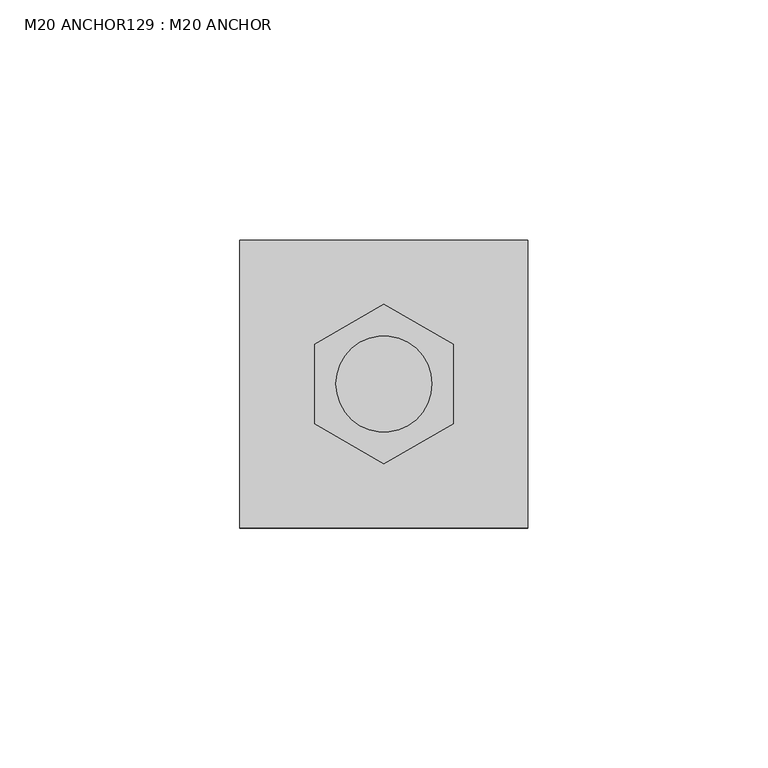
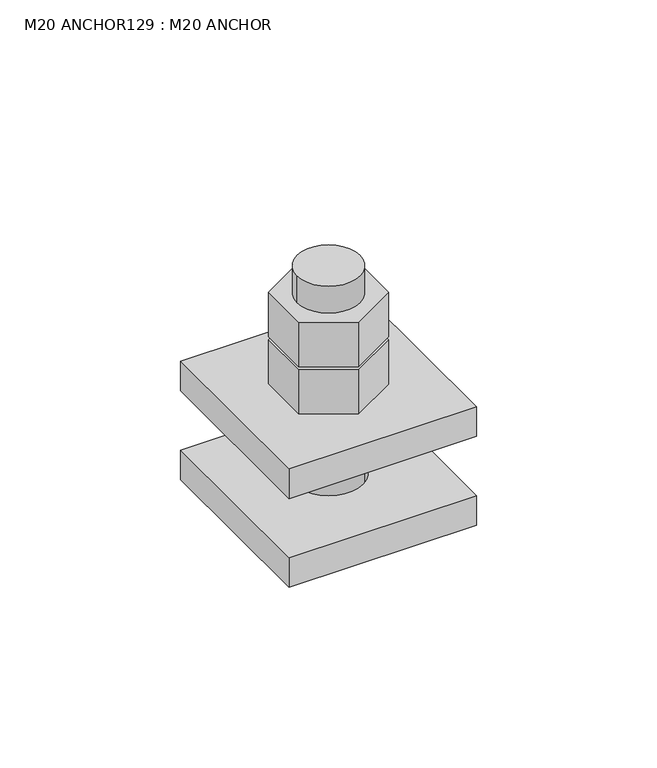
"""IFC4 building model written with IfcOpenShell, lengths in millimetres: fastener geometry, M20 ANCHOR129 : M20 ANCHOR."""

from ifc_helpers import new_model, si_unit, point, frame, frame_2d, origin, place, context, project, spatial, polyline, circle_curve, trimmed, segment, composite_curve, outline, extrude, source, transform, mapped, element, save


def m20_anchor129_m20_anchor_66062f94(model_context):
    return source(origin(), model_context, "Body", "SweptSolid", [
        extrude(outline(polyline([(5991.9144032, 19453.9464399), (5977.5062842, 19445.6279085), (5963.0981652, 19453.9464399), (5963.0981652, 19470.5835027), (5977.5062842, 19478.9020341), (5991.9144032, 19470.5835027), (5991.9144032, 19453.9464399)]), holes=[composite_curve([segment(trimmed(circle_curve(frame_2d((5977.5062842, 19462.2649713)), 10.0), [point((5967.5062842, 19462.2649713))], [point((5987.5062842, 19462.2649713))], True, "CARTESIAN"), True, "CONTINUOUS"), segment(trimmed(circle_curve(frame_2d((5977.5062842, 19462.2649713)), 10.0), [point((5987.5062842, 19462.2649713))], [point((5967.5062842, 19462.2649713))], True, "CARTESIAN"), True, "CONTINUOUS")], self_intersect=False)]), frame((0.0, 0.0, 246.0), z_axis=(0.0, 0.0, 1.0), x_axis=(1.0, 0.0, 0.0)), (0.0, 0.0, 1.0), 15.0),
        extrude(outline(polyline([(5991.9144032, 19453.9464399), (5977.5062842, 19445.6279085), (5963.0981652, 19453.9464399), (5963.0981652, 19470.5835027), (5977.5062842, 19478.9020341), (5991.9144032, 19470.5835027), (5991.9144032, 19453.9464399)]), holes=[composite_curve([segment(trimmed(circle_curve(frame_2d((5977.5062842, 19462.2649713)), 10.0), [point((5967.5062842, 19462.2649713))], [point((5987.5062842, 19462.2649713))], True, "CARTESIAN"), True, "CONTINUOUS"), segment(trimmed(circle_curve(frame_2d((5977.5062842, 19462.2649713)), 10.0), [point((5987.5062842, 19462.2649713))], [point((5967.5062842, 19462.2649713))], True, "CARTESIAN"), True, "CONTINUOUS")], self_intersect=False)]), frame((0.0, 0.0, 230.0), z_axis=(0.0, 0.0, 1.0), x_axis=(1.0, 0.0, 0.0)), (0.0, 0.0, 1.0), 15.0),
        extrude(outline(composite_curve([segment(trimmed(circle_curve(frame_2d((5977.5062842, 19462.2649713)), 10.0), [point((5967.5062842, 19462.2649713))], [point((5987.5062842, 19462.2649713))], False, "CARTESIAN"), True, "CONTINUOUS"), segment(trimmed(circle_curve(frame_2d((5977.5062842, 19462.2649713)), 10.0), [point((5987.5062842, 19462.2649713))], [point((5967.5062842, 19462.2649713))], False, "CARTESIAN"), True, "CONTINUOUS")], self_intersect=False)), frame((0.0, 0.0, 190.0), z_axis=(0.0, 0.0, 1.0), x_axis=(1.0, 0.0, 0.0)), (0.0, 0.0, 1.0), 80.0),
        extrude(outline(polyline([(6007.5062842, 19432.2649713), (5947.5062842, 19432.2649713), (5947.5062842, 19492.2649713), (6007.5062842, 19492.2649713), (6007.5062842, 19432.2649713)]), holes=[composite_curve([segment(trimmed(circle_curve(frame_2d((5977.5062842, 19462.2649713)), 11.0), [point((5966.5062842, 19462.2649713))], [point((5988.5062842, 19462.2649713))], True, "CARTESIAN"), True, "CONTINUOUS"), segment(trimmed(circle_curve(frame_2d((5977.5062842, 19462.2649713)), 11.0), [point((5988.5062842, 19462.2649713))], [point((5966.5062842, 19462.2649713))], True, "CARTESIAN"), True, "CONTINUOUS")], self_intersect=False)]), frame((0.0, 0.0, 190.0), z_axis=(0.0, 0.0, 1.0), x_axis=(1.0, 0.0, 0.0)), (0.0, 0.0, 1.0), 10.0),
        extrude(outline(polyline([(6007.5062842, 19432.2649713), (5947.5062842, 19432.2649713), (5947.5062842, 19492.2649713), (6007.5062842, 19492.2649713), (6007.5062842, 19432.2649713)]), holes=[composite_curve([segment(trimmed(circle_curve(frame_2d((5977.5062842, 19462.2649713)), 11.0), [point((5966.5062842, 19462.2649713))], [point((5988.5062842, 19462.2649713))], True, "CARTESIAN"), True, "CONTINUOUS"), segment(trimmed(circle_curve(frame_2d((5977.5062842, 19462.2649713)), 11.0), [point((5988.5062842, 19462.2649713))], [point((5966.5062842, 19462.2649713))], True, "CARTESIAN"), True, "CONTINUOUS")], self_intersect=False)]), frame((0.0, 0.0, 220.0), z_axis=(0.0, 0.0, 1.0), x_axis=(1.0, 0.0, 0.0)), (0.0, 0.0, 1.0), 10.0),
    ])


if __name__ == "__main__":
    model = new_model("IFC4")
    model_context = context("Model", 3, world=origin())
    ifc_project = project(units=[si_unit("LENGTHUNIT", "METRE", prefix="MILLI")], contexts=[model_context])
    site = spatial("IfcSite", under=ifc_project)
    building = spatial("IfcBuilding", under=site)
    placement = place(None, origin())
    m20_anchor129_m20_anchor_shape = m20_anchor129_m20_anchor_66062f94(model_context)
    element("IfcFastener", 1, ObjectType="M20 ANCHOR129 : M20 ANCHOR", at=placement, inside=building, context=model_context, shape_type="MappedRepresentation", body=[
        mapped(m20_anchor129_m20_anchor_shape, transform((0.0, 0.0, 0.0), x_axis=(1.0, 0.0, 0.0), y_axis=(0.0, 1.0, 0.0), z_axis=(0.0, 0.0, 1.0))),
    ])
    save(model, "model.ifc")
